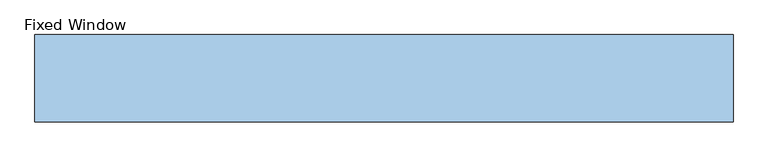
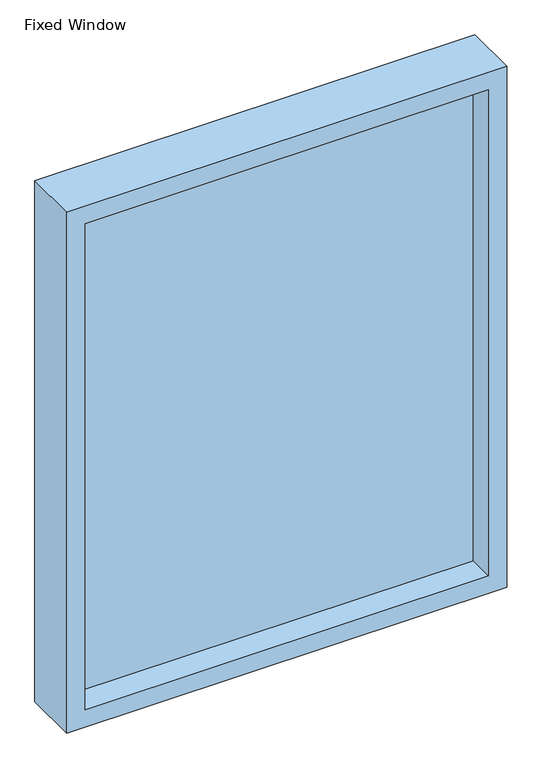
"""IFC4 building model written with IfcOpenShell, lengths in millimetres: window geometry, Fixed Window : H_WD_AR_B11_Fix_Steel Window_SG_W1200xH1500_AW-2."""

from ifc_helpers import new_model, si_unit, frame, origin, place, context, project, spatial, polyline, outline, extrude, source, transform, mapped, element, save


def fixed_window_c6e05aa5(model_context):
    return source(origin(), model_context, "Body", "SweptSolid", [
        extrude(outline(polyline([(-550.0, 3.0), (550.0, 3.0), (550.0, -3.0), (-550.0, -3.0), (-550.0, 3.0)])), frame((0.0, 0.0, 850.0), z_axis=(0.0, 0.0, 1.0), x_axis=(1.0, 0.0, 0.0)), (0.0, 0.0, 1.0), 1400.0),
        extrude(outline(polyline([(2300.0, -600.0), (800.0, -600.0), (800.0, 600.0), (2300.0, 600.0), (2300.0, -600.0)]), holes=[polyline([(2250.0, -550.0), (2250.0, 550.0), (850.0, 550.0), (850.0, -550.0), (2250.0, -550.0)])]), frame((0.0, -75.0, 0.0), z_axis=(0.0, 1.0, 0.0), x_axis=(0.0, 0.0, 1.0)), (0.0, 0.0, 1.0), 150.0),
    ])


if __name__ == "__main__":
    model = new_model("IFC4")
    model_context = context("Model", 3, world=origin())
    ifc_project = project(units=[si_unit("LENGTHUNIT", "METRE", prefix="MILLI")], contexts=[model_context])
    site = spatial("IfcSite", under=ifc_project)
    building = spatial("IfcBuilding", under=site)
    placement = place(None, origin())
    fixed_window_shape = fixed_window_c6e05aa5(model_context)
    element("IfcWindow", 1, ObjectType="Fixed Window : H_WD_AR_B11_Fix_Steel Window_SG_W1200xH1500_AW-2", at=placement, inside=building, context=model_context, shape_type="MappedRepresentation", body=[
        mapped(fixed_window_shape, transform((0.0, 0.0, 0.0), x_axis=(1.0, 0.0, 0.0), y_axis=(0.0, 1.0, 0.0), z_axis=(0.0, 0.0, 1.0))),
    ])
    save(model, "model.ifc")

# Revit data of these elements
# Type "Fixed Window : H_WD_AR_B11_Fix_Steel Window_SG_W1200xH1500_AW-2"
#   Type Mark = "269"
#   Analytic Construction = "<None>"
#   창 두께 = 150 mm
#   Height = 1500 mm
#   절반 창 두께 = 75 mm
#   기본 씰 높이 = 800 mm
#   Width = 1200 mm
#   ▽ = yes
#   Define Thermal Properties by = 1
#   창 패널 = none
#   창 프레임 = none
#   Wall Closure = (empty or 0)
#   Description = (empty or 0)
# Element 1 (IfcWindow, "Fixed Window : H_WD_AR_B11_Fix_Steel Window_SG_W1200xH1500_AW-2")
#   Materials on its faces: "00_Metal_Aluminum", "Glass"
# Materials
#   "00_Metal_Aluminum": class "Metal", colour RGB 244 244 244, transparency 0, Description = "Aluminum", Cost = 0, Image = none
#   "Glass": class "Glass", colour RGB 218 227 224, transparency 0.85, Description = "Soda Lime Glass", Cost = 0
